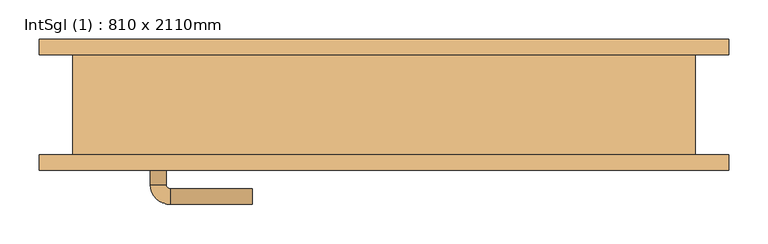
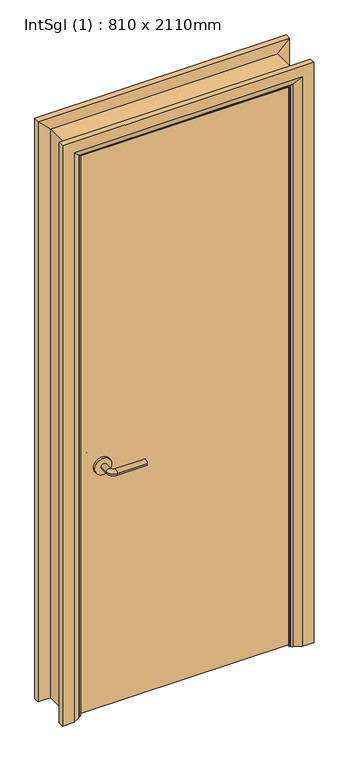
"""IFC4 building model written with IfcOpenShell, lengths in millimetres: door geometry, IntSgl (1) : 810 x 2110mm."""

import ifcopenshell
import ifcopenshell.guid

model = None  # the IFC model being written
_history = None  # IfcOwnerHistory: only IFC2X3 demands one
_inside = {}  # id of a spatial element -> (the spatial element, [elements in it])
_under = {}  # id of a project, library or spatial element -> (it, [spatial elements below it])
_declared = {}  # id of a project -> (the project, [libraries it declares])
_typed = {}  # id of a type object -> (the type object, [elements of that type])
_made_of = {}  # id of a material, layer set ... -> (it, [elements and type objects made of it])


def new_model(schema):
    """Start an empty IFC model of exactly this schema.

    Asked for "IFC4X3", IfcOpenShell would pick the latest addendum, in which some entities
    have other attributes; the version numbers below select the first issue.
    IFC2X3 requires an IfcOwnerHistory on every rooted entity: one is made here for all.
    """
    global model, _history
    if schema == "IFC4X3":
        model = ifcopenshell.file(schema_version=(4, 3, 0, 0))
    else:
        model = ifcopenshell.file(schema=schema)
    _inside.clear()
    _under.clear()
    _declared.clear()
    _typed.clear()
    _made_of.clear()
    _history = None
    if model.schema == "IFC2X3":
        org = make("IfcOrganization", Name="unknown")
        user = make(
            "IfcPersonAndOrganization",
            ThePerson=make("IfcPerson", FamilyName="unknown"),
            TheOrganization=org,
        )
        app = make(
            "IfcApplication",
            ApplicationDeveloper=org,
            Version="unknown",
            ApplicationFullName="unknown",
            ApplicationIdentifier="unknown",
        )
        _history = make(
            "IfcOwnerHistory",
            OwningUser=user,
            OwningApplication=app,
            ChangeAction="ADDED",
            CreationDate=0,
        )
    return model


def make(cls, **values):
    """One entity of the class cls with the attributes given. An attribute that is None is left unset."""
    return model.create_entity(
        cls, **{name: value for name, value in values.items() if value is not None}
    )


def rooted(cls, **values):
    """An entity with a GlobalId (a new one), such as an element, a storey or a relation."""
    return make(cls, GlobalId=ifcopenshell.guid.new(), OwnerHistory=_history, **values)


def si_unit(unit_type, name, prefix=None):
    """IfcSIUnit, for example si_unit("LENGTHUNIT", "METRE", prefix="MILLI")."""
    return make("IfcSIUnit", UnitType=unit_type, Prefix=prefix, Name=name)


def assignment(units):
    """IfcUnitAssignment: the units of a project."""
    return None if units is None else make("IfcUnitAssignment", Units=units)


def point(xyz):
    """IfcCartesianPoint."""
    return None if xyz is None else make("IfcCartesianPoint", Coordinates=xyz)


def direction(xyz):
    """IfcDirection."""
    return None if xyz is None else make("IfcDirection", DirectionRatios=xyz)


def frame(location, z_axis=None, x_axis=None):
    """IfcAxis2Placement3D, a coordinate frame: its origin and axes. An axis left out is left unset."""
    return make(
        "IfcAxis2Placement3D",
        Location=point(location),
        Axis=direction(z_axis),
        RefDirection=direction(x_axis),
    )


def frame_2d(location, x_axis=None):
    """IfcAxis2Placement2D, a coordinate frame in the plane: its origin and x axis."""
    return make(
        "IfcAxis2Placement2D", Location=point(location), RefDirection=direction(x_axis)
    )


def origin():
    """The frame at (0, 0, 0) with its axes left unset."""
    return frame((0.0, 0.0, 0.0))


def place(relative_to, where):
    """IfcLocalPlacement: puts the frame where relative to a parent placement (None: the world)."""
    return make(
        "IfcLocalPlacement", PlacementRelTo=relative_to, RelativePlacement=where
    )


def context(
    kind, dimensions, precision=None, world=None, true_north=None, identifier=None
):
    """IfcGeometricRepresentationContext, for example the 3D "Model" context."""
    return make(
        "IfcGeometricRepresentationContext",
        ContextIdentifier=identifier,
        ContextType=kind,
        CoordinateSpaceDimension=dimensions,
        Precision=precision,
        WorldCoordinateSystem=world,
        TrueNorth=true_north,
    )


def project(units=None, contexts=None):
    """IfcProject with its units and contexts."""
    return rooted(
        "IfcProject",
        Name="project",
        RepresentationContexts=contexts,
        UnitsInContext=assignment(units),
    )


def spatial(cls, under=None, at=None, **own):
    """A site, building, storey or space (cls), placed at a placement, below another one or the project."""
    s = rooted(cls, ObjectPlacement=at, **own)
    if under is not None:
        _under.setdefault(under.id(), (under, []))[1].append(s)
    return s


def polyline(points):
    """IfcPolyline through the points."""
    return make("IfcPolyline", Points=[point(p) for p in points])


def circle_curve(where, radius):
    """IfcCircle in the frame where."""
    return make("IfcCircle", Position=where, Radius=radius)


def ellipse_curve(where, semi_axis1, semi_axis2):
    """IfcEllipse in the frame where."""
    return make(
        "IfcEllipse", Position=where, SemiAxis1=semi_axis1, SemiAxis2=semi_axis2
    )


def trimmed(basis, trim1, trim2, sense, master):
    """IfcTrimmedCurve: the piece of a basis curve between two trims."""
    return make(
        "IfcTrimmedCurve",
        BasisCurve=basis,
        Trim1=trim1,
        Trim2=trim2,
        SenseAgreement=sense,
        MasterRepresentation=master,
    )


def segment(curve, same_sense, transition):
    """IfcCompositeCurveSegment."""
    return make(
        "IfcCompositeCurveSegment",
        Transition=transition,
        SameSense=same_sense,
        ParentCurve=curve,
    )


def composite_curve(segments, self_intersect=None):
    """IfcCompositeCurve: segments joined end to end."""
    return make("IfcCompositeCurve", Segments=segments, SelfIntersect=self_intersect)


def outline(outer, holes=None, kind="AREA"):
    """IfcArbitraryClosedProfileDef: a profile drawn as a closed curve; with holes, ...WithVoids."""
    if holes is None:
        return make("IfcArbitraryClosedProfileDef", ProfileType=kind, OuterCurve=outer)
    return make(
        "IfcArbitraryProfileDefWithVoids",
        ProfileType=kind,
        OuterCurve=outer,
        InnerCurves=holes,
    )


def extrude(swept, where, along, depth):
    """IfcExtrudedAreaSolid: the profile swept, set in the frame where, extruded along a direction by depth."""
    return make(
        "IfcExtrudedAreaSolid",
        SweptArea=swept,
        Position=where,
        ExtrudedDirection=direction(along),
        Depth=depth,
    )


def faces_of(points, faces, orient=None, outer=None):
    """IfcFace entities. A face is a list of loops; a loop is a list of indices into points, from 0.

    orient and outer hold one flag for each loop. By default every Orientation is true, the
    first loop of a face is its IfcFaceOuterBound and the others are IfcFaceBound.
    """
    made = []
    for i, loops in enumerate(faces):
        bounds = []
        for j, loop in enumerate(loops):
            is_outer = j == 0 if outer is None else outer[i][j]
            bounds.append(
                make(
                    "IfcFaceOuterBound" if is_outer else "IfcFaceBound",
                    Bound=make("IfcPolyLoop", Polygon=[points[k] for k in loop]),
                    Orientation=True if orient is None else orient[i][j],
                )
            )
        made.append(make("IfcFace", Bounds=bounds))
    return made


def faceted_brep(points, faces, orient=None, outer=None, voids=None):
    """IfcFacetedBrep: a solid bounded by flat faces; with voids (closed shells), ...WithVoids."""
    shared = [point(p) for p in points]
    hull = make("IfcClosedShell", CfsFaces=faces_of(shared, faces, orient, outer))
    if voids is None:
        return make("IfcFacetedBrep", Outer=hull)
    return make(
        "IfcFacetedBrepWithVoids",
        Outer=hull,
        Voids=[
            make(cls, CfsFaces=faces_of(shared, fs, o, b)) for cls, fs, o, b in voids
        ],
    )


def shape(context_of_items, identifier, shape_type, items):
    """IfcShapeRepresentation: the items that make up one representation, for example the "Body"."""
    return make(
        "IfcShapeRepresentation",
        ContextOfItems=context_of_items,
        RepresentationIdentifier=identifier,
        RepresentationType=shape_type,
        Items=items,
    )


def source(mapping_origin, context_of_items, identifier, shape_type, items):
    """IfcRepresentationMap: a shape defined once, which mapped items show again and again."""
    return make(
        "IfcRepresentationMap",
        MappingOrigin=mapping_origin,
        MappedRepresentation=shape(context_of_items, identifier, shape_type, items),
    )


def transform(
    local_origin,
    x_axis=None,
    y_axis=None,
    z_axis=None,
    scale=None,
    scale2=None,
    scale3=None,
    uniform=True,
):
    """IfcCartesianTransformationOperator3D, or its non-uniform kind. x_axis, y_axis, z_axis: its Axis1, 2, 3."""
    if uniform:
        return make(
            "IfcCartesianTransformationOperator3D",
            Axis1=direction(x_axis),
            Axis2=direction(y_axis),
            LocalOrigin=point(local_origin),
            Scale=scale,
            Axis3=direction(z_axis),
        )
    return make(
        "IfcCartesianTransformationOperator3DnonUniform",
        Axis1=direction(x_axis),
        Axis2=direction(y_axis),
        LocalOrigin=point(local_origin),
        Scale=scale,
        Axis3=direction(z_axis),
        Scale2=scale2,
        Scale3=scale3,
    )


def mapped(mapping_source, mapping_target):
    """IfcMappedItem: shows the shape of a source again, moved by a transform."""
    return make(
        "IfcMappedItem", MappingSource=mapping_source, MappingTarget=mapping_target
    )


def made_of(thing, what):
    """Note that an element or type object is made of a material, layer set ...; save() writes the relation."""
    if what is not None:
        _made_of.setdefault(what.id(), (what, []))[1].append(thing)
    return thing


def element(
    cls,
    number,
    at=None,
    inside=None,
    cuts=None,
    type_object=None,
    material=None,
    context=None,
    identifier="Body",
    shape_type=None,
    held_by="IfcProductDefinitionShape",
    body=None,
    shapes=None,
    **own,
):
    """One element of the class cls, such as IfcWall. Its Tag is "e" and its number.

    at: its placement. inside: the storey or other place that contains it. cuts: it is an
    opening in that element (IfcRelVoidsElement). A single representation is given by context,
    identifier, shape_type and body (its items); several are given by shapes. held_by: the class
    of the entity that holds the representations. save() writes the other relations.
    """
    e = rooted(cls, Tag="e%d" % number, ObjectPlacement=at, **own)
    if body is not None:
        shapes = [shape(context, identifier, shape_type, body)]
    if shapes is not None:
        e.Representation = make(held_by, Representations=shapes)
    if inside is not None:
        _inside.setdefault(inside.id(), (inside, []))[1].append(e)
    if cuts is not None:
        rooted(
            "IfcRelVoidsElement", RelatingBuildingElement=cuts, RelatedOpeningElement=e
        )
    if type_object is not None:
        _typed.setdefault(type_object.id(), (type_object, []))[1].append(e)
    return made_of(e, material)


def aggregate(whole, parts):
    """IfcRelAggregates: a whole, such as a stair, and the parts it consists of."""
    return rooted("IfcRelAggregates", RelatingObject=whole, RelatedObjects=parts)


def save(model, path):
    """Write the relations noted so far, then the file.

    IfcRelAggregates (storeys below a building ...), IfcRelContainedInSpatialStructure (elements
    in a storey), IfcRelDefinesByType, IfcRelAssociatesMaterial and IfcRelDeclares: one each for
    every whole, place, type object, material and project.
    """
    for whole, parts in _under.values():
        aggregate(whole, parts)
    for where, things in _inside.values():
        rooted(
            "IfcRelContainedInSpatialStructure",
            RelatedElements=things,
            RelatingStructure=where,
        )
    for kind, things in _typed.values():
        rooted("IfcRelDefinesByType", RelatedObjects=things, RelatingType=kind)
    for what, things in _made_of.values():
        rooted("IfcRelAssociatesMaterial", RelatedObjects=things, RelatingMaterial=what)
    for by, libraries in _declared.values():
        rooted("IfcRelDeclares", RelatingContext=by, RelatedDefinitions=libraries)
    model.write(path)


def plane_surface(at):
    """IfcPlane: the flat surface through the origin of the frame at, square to its z axis."""
    return make("IfcPlane", Position=at)


def cylinder_surface(at, radius):
    """IfcCylindricalSurface: all points at the distance radius from the z axis of the frame at."""
    return make("IfcCylindricalSurface", Position=at, Radius=radius)


def revolved_surface(curve, axis_point, axis_direction):
    """IfcSurfaceOfRevolution: the curve turned about the line through axis_point along axis_direction."""
    return make(
        "IfcSurfaceOfRevolution",
        SweptCurve=make("IfcArbitraryOpenProfileDef", ProfileType="CURVE", Curve=curve),
        AxisPosition=make("IfcAxis1Placement", Location=point(axis_point), Axis=direction(axis_direction)),
    )


def advanced_brep(points, edges, surfaces, faces):
    """IfcAdvancedBrep: a solid bounded by faces that lie on surfaces and meet in shared edges.

    An edge is (start, end): straight between two places in points (the first is 0);
    or (start, end, curve); or (start, end, curve, False) where it runs against its curve.
    A face is (place in surfaces, loops), or (place, loops, False) where it looks against
    its surface's normal. A loop lists edges by number (the first is 1), with a minus sign
    where the edge is run from its end to its start. The first loop is the outer one.
    """
    corners = [point(p) for p in points]
    vertices = [make("IfcVertexPoint", VertexGeometry=c) for c in corners]
    made = []
    for start, end, *more in edges:
        made.append(
            make(
                "IfcEdgeCurve",
                EdgeStart=vertices[start],
                EdgeEnd=vertices[end],
                EdgeGeometry=more[0] if more else make("IfcPolyline", Points=[corners[start], corners[end]]),
                SameSense=more[1] if len(more) > 1 else True,
            )
        )
    hull = []
    for where, loops, *sense in faces:
        bounds = []
        for j, loop in enumerate(loops):
            ring = [make("IfcOrientedEdge", EdgeElement=made[abs(k) - 1], Orientation=k > 0) for k in loop]
            bounds.append(
                make(
                    "IfcFaceOuterBound" if j == 0 else "IfcFaceBound",
                    Bound=make("IfcEdgeLoop", EdgeList=ring),
                    Orientation=True,
                )
            )
        hull.append(make("IfcAdvancedFace", Bounds=bounds, FaceSurface=surfaces[where], SameSense=sense[0] if sense else True))
    return make("IfcAdvancedBrep", Outer=make("IfcClosedShell", CfsFaces=hull))


def intsgl_1_810_x_2110mm_198b6b43(model_context):
    return source(origin(), model_context, "Body", "SolidModel", [
        advanced_brep(
        [(-298.0, -17.75, 900.0), (-278.0, -17.75, 900.0), (-298.0, 12.25, 900.0), (-278.0, 12.25, 900.0), (-273.0, 17.25, 900.0), (-273.0, 37.25, 900.0), (-168.0, 37.25, 900.0), (-168.0, 17.25, 900.0)],
        [
            (0, 1, circle_curve(frame((-288.0, -17.75, 900.0), z_axis=(0.0, -1.0, 0.0), x_axis=(1.0, 0.0, 0.0)), 10.0)),
            (1, 0, circle_curve(frame((-288.0, -17.75, 900.0), z_axis=(0.0, -1.0, 0.0), x_axis=(1.0, 0.0, 0.0)), 10.0)),
            (0, 2),
            (2, 3, circle_curve(frame((-288.0, 12.25, 900.0), z_axis=(0.0, -1.0, 0.0), x_axis=(1.0, 0.0, 0.0)), 10.0)),
            (3, 1),
            (3, 2, circle_curve(frame((-288.0, 12.25, 900.0), z_axis=(0.0, -1.0, 0.0), x_axis=(1.0, 0.0, 0.0)), 10.0)),
            (4, 3, circle_curve(frame((-273.0, 12.25, 900.0), z_axis=(0.0, 0.0, 1.0), x_axis=(-1.0, 0.0, 0.0)), 5.0)),
            (2, 5, circle_curve(frame((-273.0, 12.25, 900.0), z_axis=(0.0, 0.0, -1.0), x_axis=(-1.0, 0.0, 0.0)), 25.0)),
            (5, 4, circle_curve(frame((-273.0, 27.25, 900.0), z_axis=(-1.0, 0.0, 0.0), x_axis=(0.0, -1.0, 0.0)), 10.0)),
            (4, 5, circle_curve(frame((-273.0, 27.25, 900.0), z_axis=(-1.0, 0.0, 0.0), x_axis=(0.0, -1.0, 0.0)), 10.0)),
            (6, 7, circle_curve(frame((-168.0, 27.25, 900.0), z_axis=(1.0, 0.0, 0.0), x_axis=(0.0, -1.0, 0.0)), 10.0)),
            (7, 6, circle_curve(frame((-168.0, 27.25, 900.0), z_axis=(1.0, 0.0, 0.0), x_axis=(0.0, -1.0, 0.0)), 10.0)),
            (5, 6),
            (7, 4),
        ],
        [
            plane_surface(frame((-288.0, -17.75, 900.0), z_axis=(0.0, -1.0, 0.0), x_axis=(0.0, 0.0, 1.0))),
            cylinder_surface(frame((-288.0, -17.75, 900.0), z_axis=(0.0, -1.0, 0.0), x_axis=(1.0, 0.0, 0.0)), 10.0),
            revolved_surface(trimmed(ellipse_curve(frame((-288.0, 12.25, 900.0), z_axis=(0.0, -1.0, 0.0), x_axis=(1.0, 0.0, 0.0)), 10.0, 10.0), [point((-298.0, 12.25, 900.0))], [point((-278.0, 12.25, 900.0))], True, "CARTESIAN"), (-273.0, 12.25, 900.0), (0.0, 0.0, -1.0)),
            revolved_surface(trimmed(ellipse_curve(frame((-288.0, 12.25, 900.0), z_axis=(0.0, -1.0, 0.0), x_axis=(1.0, 0.0, 0.0)), 10.0, 10.0), [point((-278.0, 12.25, 900.0))], [point((-298.0, 12.25, 900.0))], True, "CARTESIAN"), (-273.0, 12.25, 900.0), (0.0, 0.0, -1.0)),
            plane_surface(frame((-168.0, 27.25, 900.0), z_axis=(1.0, 0.0, 0.0), x_axis=(0.0, 0.0, 1.0))),
            cylinder_surface(frame((-273.0, 27.25, 900.0), z_axis=(-1.0, 0.0, 0.0), x_axis=(0.0, -1.0, 0.0)), 10.0),
        ],
        [
            (0, [[1, 2]]),
            (1, [[-1, 3, 4, 5]]),
            (1, [[-2, -5, 6, -3]]),
            (2, [[7, -4, 8, 9]]),
            (3, [[-8, -6, -7, 10]]),
            (4, [[11, 12]]),
            (5, [[-9, 13, -12, 14]]),
            (5, [[-10, -14, -11, -13]]),
        ],
    ),
        extrude(outline(composite_curve([segment(trimmed(circle_curve(frame_2d((900.0, -290.5)), 30.0), [point((900.0, -320.5))], [point((900.0, -260.5))], False, "CARTESIAN"), True, "CONTINUOUS"), segment(trimmed(circle_curve(frame_2d((900.0, -290.5)), 30.0), [point((900.0, -260.5))], [point((900.0, -320.5))], False, "CARTESIAN"), True, "CONTINUOUS")], self_intersect=False)), frame((0.0, -25.75, 0.0), z_axis=(0.0, 1.0, 0.0), x_axis=(0.0, 0.0, 1.0)), (0.0, 0.0, 1.0), 8.0),
        advanced_brep(
        [(-298.0, -71.75, 900.0), (-278.0, -71.75, 900.0), (-278.0, -101.75, 900.0), (-298.0, -101.75, 900.0), (-273.0, -106.75, 900.0), (-273.0, -126.75, 900.0), (-168.0, -126.75, 900.0), (-168.0, -106.75, 900.0)],
        [
            (0, 1, circle_curve(frame((-288.0, -71.75, 900.0), z_axis=(0.0, 1.0, 0.0), x_axis=(1.0, 0.0, 0.0)), 10.0)),
            (1, 0, circle_curve(frame((-288.0, -71.75, 900.0), z_axis=(0.0, 1.0, 0.0), x_axis=(1.0, 0.0, 0.0)), 10.0)),
            (1, 2),
            (2, 3, circle_curve(frame((-288.0, -101.75, 900.0), z_axis=(0.0, 1.0, 0.0), x_axis=(1.0, 0.0, 0.0)), 10.0)),
            (3, 0),
            (3, 2, circle_curve(frame((-288.0, -101.75, 900.0), z_axis=(0.0, 1.0, 0.0), x_axis=(1.0, 0.0, 0.0)), 10.0)),
            (4, 5, circle_curve(frame((-273.0, -116.75, 900.0), z_axis=(-1.0, 0.0, 0.0), x_axis=(0.0, 1.0, 0.0)), 10.0)),
            (5, 3, circle_curve(frame((-273.0, -101.75, 900.0), z_axis=(0.0, 0.0, -1.0), x_axis=(-1.0, 0.0, 0.0)), 25.0)),
            (2, 4, circle_curve(frame((-273.0, -101.75, 900.0), z_axis=(0.0, 0.0, 1.0), x_axis=(-1.0, 0.0, 0.0)), 5.0)),
            (5, 4, circle_curve(frame((-273.0, -116.75, 900.0), z_axis=(-1.0, 0.0, 0.0), x_axis=(0.0, 1.0, 0.0)), 10.0)),
            (6, 7, circle_curve(frame((-168.0, -116.75, 900.0), z_axis=(1.0, 0.0, 0.0), x_axis=(0.0, 1.0, 0.0)), 10.0)),
            (7, 6, circle_curve(frame((-168.0, -116.75, 900.0), z_axis=(1.0, 0.0, 0.0), x_axis=(0.0, 1.0, 0.0)), 10.0)),
            (4, 7),
            (6, 5),
        ],
        [
            plane_surface(frame((-288.0, -71.75, 900.0), z_axis=(0.0, 1.0, 0.0), x_axis=(0.0, 0.0, 1.0))),
            cylinder_surface(frame((-288.0, -71.75, 900.0), z_axis=(0.0, 1.0, 0.0), x_axis=(1.0, 0.0, 0.0)), 10.0),
            revolved_surface(trimmed(ellipse_curve(frame((-288.0, -101.75, 900.0), z_axis=(0.0, -1.0, 0.0), x_axis=(1.0, 0.0, 0.0)), 10.0, 10.0), [point((-298.0, -101.75, 900.0))], [point((-278.0, -101.75, 900.0))], True, "CARTESIAN"), (-273.0, -101.75, 900.0), (0.0, 0.0, -1.0)),
            revolved_surface(trimmed(ellipse_curve(frame((-288.0, -101.75, 900.0), z_axis=(0.0, -1.0, 0.0), x_axis=(1.0, 0.0, 0.0)), 10.0, 10.0), [point((-278.0, -101.75, 900.0))], [point((-298.0, -101.75, 900.0))], True, "CARTESIAN"), (-273.0, -101.75, 900.0), (0.0, 0.0, -1.0)),
            plane_surface(frame((-168.0, -116.75, 900.0), z_axis=(1.0, 0.0, 0.0), x_axis=(0.0, 0.0, 1.0))),
            cylinder_surface(frame((-273.0, -116.75, 900.0), z_axis=(-1.0, 0.0, 0.0), x_axis=(0.0, 1.0, 0.0)), 10.0),
        ],
        [
            (0, [[1, 2]]),
            (1, [[3, 4, 5, -2]]),
            (1, [[-5, 6, -3, -1]]),
            (2, [[7, 8, -4, 9]]),
            (3, [[10, -9, -6, -8]]),
            (4, [[11, 12]]),
            (5, [[13, -11, 14, -7]]),
            (5, [[-14, -12, -13, -10]]),
        ],
    ),
        extrude(outline(composite_curve([segment(trimmed(circle_curve(frame_2d((900.0, -290.5)), 30.0), [point((900.0, -320.5))], [point((900.0, -260.5))], False, "CARTESIAN"), True, "CONTINUOUS"), segment(trimmed(circle_curve(frame_2d((900.0, -290.5)), 30.0), [point((900.0, -260.5))], [point((900.0, -320.5))], False, "CARTESIAN"), True, "CONTINUOUS")], self_intersect=False)), frame((0.0, -71.75, 0.0), z_axis=(0.0, 1.0, 0.0), x_axis=(0.0, 0.0, 1.0)), (0.0, 0.0, 1.0), 8.0),
        extrude(outline(polyline([(363.0, -25.75), (363.0, -63.75), (-363.0, -63.75), (-363.0, -25.75), (363.0, -25.75)])), frame((0.0, 0.0, 8.0), z_axis=(0.0, 0.0, 1.0), x_axis=(1.0, 0.0, 0.0)), (0.0, 0.0, 1.0), 2060.0),
        advanced_brep(
        [(440.0, -83.75, 0.0), (400.0, -83.75, 0.0), (374.0, -69.75, 0.0), (370.0, -63.75, 0.0), (440.0, -63.75, 0.0), (440.0, -63.75, 2145.0), (440.0, -83.75, 2145.0), (370.0, -63.75, 2075.0), (-370.0, -63.75, 2075.0), (-370.0, -63.75, 0.0), (-440.0, -63.75, 0.0), (-440.0, -63.75, 2145.0), (374.0, -69.75, 2079.0), (400.0, -83.75, 2105.0), (-440.0, -83.75, 2145.0), (-440.0, -83.75, 0.0), (-400.0, -83.75, 0.0), (-400.0, -83.75, 2105.0), (-374.0, -69.75, 2079.0), (-374.0, -69.75, 0.0)],
        [
            (0, 1),
            (1, 2),
            (2, 3, circle_curve(frame((378.0, -62.75, 0.0), z_axis=(0.0, 0.0, -1.0), x_axis=(1.0, 0.0, 0.0)), 8.0622577)),
            (3, 4),
            (4, 0),
            (4, 5),
            (5, 6),
            (6, 0),
            (3, 7),
            (7, 8),
            (8, 9),
            (9, 10),
            (10, 11),
            (11, 5),
            (2, 12),
            (12, 7, ellipse_curve(frame((378.0, -62.75, 2083.0), z_axis=(0.7071067811865475, 0.0, -0.7071067811865475), x_axis=(-0.7071067811865474, 0.0, -0.7071067811865476)), 11.4017543, 8.0622577)),
            (1, 13),
            (13, 12),
            (6, 14),
            (14, 15),
            (15, 16),
            (16, 17),
            (17, 13),
            (11, 14),
            (12, 18),
            (18, 8, ellipse_curve(frame((-378.0, -62.75, 2083.0), z_axis=(0.7071067811865475, 0.0, 0.7071067811865475), x_axis=(0.7071067811865476, 0.0, -0.7071067811865474)), 11.4017543, 8.0622577)),
            (17, 18),
            (15, 10),
            (9, 19, circle_curve(frame((-378.0, -62.75, 0.0), z_axis=(0.0, 0.0, -1.0), x_axis=(-1.0, 0.0, 0.0)), 8.0622577)),
            (19, 16),
            (18, 19),
        ],
        [
            plane_surface(frame((370.0, -63.75, 0.0), z_axis=(0.0, 0.0, -1.0), x_axis=(0.0, 1.0, 0.0))),
            plane_surface(frame((440.0, -83.75, 0.0), z_axis=(1.0, 0.0, 0.0), x_axis=(0.0, 0.0, 1.0))),
            plane_surface(frame((440.0, -63.75, 0.0), z_axis=(0.0, 1.0, 0.0), x_axis=(0.0, 0.0, 1.0))),
            cylinder_surface(frame((378.0, -62.75, 0.0), z_axis=(0.0, 0.0, -1.0), x_axis=(1.0, 0.0, 0.0)), 8.0622577),
            plane_surface(frame((374.0, -69.75, 0.0), z_axis=(-0.4740998230350126, -0.880471099922178, 0.0), x_axis=(0.0, 0.0, 1.0))),
            plane_surface(frame((400.0, -83.75, 0.0), z_axis=(0.0, -1.0, 0.0), x_axis=(0.0, 0.0, 1.0))),
            plane_surface(frame((440.0, -83.75, 2145.0), z_axis=(0.0, 0.0, 1.0), x_axis=(-1.0, 0.0, 0.0))),
            cylinder_surface(frame((370.0, -62.75, 2083.0), z_axis=(1.0, 0.0, 0.0), x_axis=(0.0, 0.0, 1.0)), 8.0622577),
            plane_surface(frame((374.0, -69.75, 2079.0), z_axis=(0.0, -0.8804710999221764, -0.4740998230350154), x_axis=(-1.0, 0.0, 0.0))),
            plane_surface(frame((-370.0, -63.75, 0.0), z_axis=(0.0, 0.0, -1.0), x_axis=(0.0, 1.0, 0.0))),
            plane_surface(frame((-440.0, -83.75, 2145.0), z_axis=(-1.0, 0.0, 0.0), x_axis=(0.0, 0.0, -1.0))),
            cylinder_surface(frame((-378.0, -62.75, 2075.0), z_axis=(0.0, 0.0, 1.0), x_axis=(-1.0, 0.0, 0.0)), 8.0622577),
            plane_surface(frame((-374.0, -69.75, 2079.0), z_axis=(0.47409982303501824, -0.8804710999221749, 0.0), x_axis=(0.0, 0.0, -1.0))),
        ],
        [
            (0, [[1, 2, 3, 4, 5]]),
            (1, [[6, 7, 8, -5]]),
            (2, [[9, 10, 11, 12, 13, 14, -6, -4]]),
            (3, [[15, 16, -9, -3]]),
            (4, [[17, 18, -15, -2]]),
            (5, [[-8, 19, 20, 21, 22, 23, -17, -1]]),
            (6, [[-14, 24, -19, -7]]),
            (7, [[25, 26, -10, -16]]),
            (8, [[-23, 27, -25, -18]]),
            (9, [[28, -12, 29, 30, -21]]),
            (10, [[-13, -28, -20, -24]]),
            (11, [[31, -29, -11, -26]]),
            (12, [[-22, -30, -31, -27]]),
        ],
    ),
        extrude(outline(polyline([(0.0, -346.0), (2051.0, -346.0), (2051.0, 346.0), (0.0, 346.0), (0.0, 365.0), (2070.0, 365.0), (2070.0, -365.0), (0.0, -365.0), (0.0, -346.0)])), frame((0.0, -23.75, 0.0), z_axis=(0.0, 1.0, 0.0), x_axis=(0.0, 0.0, 1.0)), (0.0, 0.0, 1.0), 32.0),
        advanced_brep(
        [(-440.0, 83.75, 0.0), (-400.0, 83.75, 0.0), (-374.0, 69.75, 0.0), (-370.0, 63.75, 0.0), (-440.0, 63.75, 0.0), (-440.0, 63.75, 2145.0), (-440.0, 83.75, 2145.0), (-370.0, 63.75, 2075.0), (-374.0, 69.75, 2079.0), (-400.0, 83.75, 2105.0), (440.0, 63.75, 2145.0), (440.0, 83.75, 2145.0), (370.0, 63.75, 2075.0), (374.0, 69.75, 2079.0), (400.0, 83.75, 2105.0), (440.0, 83.75, 0.0), (440.0, 63.75, 0.0), (370.0, 63.75, 0.0), (374.0, 69.75, 0.0), (400.0, 83.75, 0.0)],
        [
            (0, 1),
            (1, 2),
            (2, 3, circle_curve(frame((-378.0, 62.75, 0.0), z_axis=(0.0, 0.0, -1.0), x_axis=(-1.0, 0.0, 0.0)), 8.0622577)),
            (3, 4),
            (4, 0),
            (4, 5),
            (5, 6),
            (6, 0),
            (3, 7),
            (7, 5),
            (2, 8),
            (8, 7, ellipse_curve(frame((-378.0, 62.75, 2083.0), z_axis=(-0.7071067811865475, 0.0, -0.7071067811865475), x_axis=(0.7071067811865474, 0.0, -0.7071067811865476)), 11.4017543, 8.0622577)),
            (1, 9),
            (9, 8),
            (6, 9),
            (5, 10),
            (10, 11),
            (11, 6),
            (7, 12),
            (12, 10),
            (8, 13),
            (13, 12, ellipse_curve(frame((378.0, 62.75, 2083.0), z_axis=(-0.7071067811865475, 0.0, 0.7071067811865475), x_axis=(-0.7071067811865476, 0.0, -0.7071067811865474)), 11.4017543, 8.0622577)),
            (9, 14),
            (14, 13),
            (11, 14),
            (15, 16),
            (16, 17),
            (17, 18, circle_curve(frame((378.0, 62.75, 0.0), z_axis=(0.0, 0.0, -1.0), x_axis=(1.0, 0.0, 0.0)), 8.0622577)),
            (18, 19),
            (19, 15),
            (10, 16),
            (15, 11),
            (12, 17),
            (13, 18),
            (14, 19),
        ],
        [
            plane_surface(frame((-370.0, 136.5510989, 0.0), z_axis=(0.0, 0.0, -1.0), x_axis=(1.0, 0.0, 0.0))),
            plane_surface(frame((-440.0, 83.75, 0.0), z_axis=(-1.0, 0.0, 0.0), x_axis=(0.0, 0.0, 1.0))),
            plane_surface(frame((-440.0, 63.75, 0.0), z_axis=(0.0, -1.0, 0.0), x_axis=(0.0, 0.0, 1.0))),
            cylinder_surface(frame((-378.0, 62.75, 0.0), z_axis=(0.0, 0.0, -1.0), x_axis=(-1.0, 0.0, 0.0)), 8.0622577),
            plane_surface(frame((-374.0, 69.75, 0.0), z_axis=(0.4740998230350183, 0.8804710999221749, 0.0), x_axis=(0.0, 0.0, 1.0))),
            plane_surface(frame((-400.0, 83.75, 0.0), z_axis=(0.0, 1.0, 0.0), x_axis=(0.0, 0.0, 1.0))),
            plane_surface(frame((-440.0, 83.75, 2145.0), z_axis=(0.0, 0.0, 1.0), x_axis=(1.0, 0.0, 0.0))),
            plane_surface(frame((-440.0, 63.75, 2145.0), z_axis=(0.0, -1.0, 0.0), x_axis=(1.0, 0.0, 0.0))),
            cylinder_surface(frame((-370.0, 62.75, 2083.0), z_axis=(-1.0, 0.0, 0.0), x_axis=(0.0, 0.0, 1.0)), 8.0622577),
            plane_surface(frame((-374.0, 69.75, 2079.0), z_axis=(0.0, 0.8804710999221749, -0.4740998230350183), x_axis=(1.0, 0.0, 0.0))),
            plane_surface(frame((-400.0, 83.75, 2105.0), z_axis=(0.0, 1.0, 0.0), x_axis=(1.0, 0.0, 0.0))),
            plane_surface(frame((370.0, 136.5510989, 0.0), z_axis=(0.0, 0.0, -1.0), x_axis=(-1.0, 0.0, 0.0))),
            plane_surface(frame((440.0, 83.75, 2145.0), z_axis=(1.0, 0.0, 0.0), x_axis=(0.0, 0.0, -1.0))),
            plane_surface(frame((440.0, 63.75, 2145.0), z_axis=(0.0, -1.0, 0.0), x_axis=(0.0, 0.0, -1.0))),
            cylinder_surface(frame((378.0, 62.75, 2075.0), z_axis=(0.0, 0.0, 1.0), x_axis=(1.0, 0.0, 0.0)), 8.0622577),
            plane_surface(frame((374.0, 69.75, 2079.0), z_axis=(-0.4740998230350183, 0.8804710999221749, 0.0), x_axis=(0.0, 0.0, -1.0))),
            plane_surface(frame((400.0, 83.75, 2105.0), z_axis=(0.0, 1.0, 0.0), x_axis=(0.0, 0.0, -1.0))),
        ],
        [
            (0, [[1, 2, 3, 4, 5]]),
            (1, [[6, 7, 8, -5]]),
            (2, [[9, 10, -6, -4]]),
            (3, [[11, 12, -9, -3]]),
            (4, [[13, 14, -11, -2]]),
            (5, [[-8, 15, -13, -1]]),
            (6, [[16, 17, 18, -7]]),
            (7, [[19, 20, -16, -10]]),
            (8, [[21, 22, -19, -12]]),
            (9, [[23, 24, -21, -14]]),
            (10, [[-18, 25, -23, -15]]),
            (11, [[26, 27, 28, 29, 30]]),
            (12, [[31, -26, 32, -17]]),
            (13, [[33, -27, -31, -20]]),
            (14, [[34, -28, -33, -22]]),
            (15, [[35, -29, -34, -24]]),
            (16, [[-32, -30, -35, -25]]),
        ],
    ),
        faceted_brep([(-365.0, -63.75, 0.0), (-397.0, -63.75, 0.0), (-397.0, 63.75, 0.0), (-365.0, 63.75, 0.0), (-365.0, 63.75, 2070.0), (-365.0, -63.75, 2070.0), (-397.0, 63.75, 2102.0), (-397.0, -63.75, 2102.0), (365.0, 63.75, 2070.0), (365.0, -63.75, 2070.0), (397.0, 63.75, 2102.0), (397.0, -63.75, 2102.0), (365.0, -63.75, 0.0), (365.0, 63.75, 0.0), (397.0, 63.75, 0.0), (397.0, -63.75, 0.0)], [[[0, 1, 2, 3]], [[3, 4, 5, 0]], [[2, 6, 4, 3]], [[1, 7, 6, 2]], [[0, 5, 7, 1]], [[4, 8, 9, 5]], [[6, 10, 8, 4]], [[7, 11, 10, 6]], [[5, 9, 11, 7]], [[12, 13, 14, 15]], [[8, 13, 12, 9]], [[10, 14, 13, 8]], [[11, 15, 14, 10]], [[9, 12, 15, 11]]]),
    ])


if __name__ == "__main__":
    model = new_model("IFC4")
    model_context = context("Model", 3, world=origin())
    ifc_project = project(units=[si_unit("LENGTHUNIT", "METRE", prefix="MILLI")], contexts=[model_context])
    site = spatial("IfcSite", under=ifc_project)
    building = spatial("IfcBuilding", under=site)
    placement = place(None, origin())
    intsgl_1_810_x_2110mm_shape = intsgl_1_810_x_2110mm_198b6b43(model_context)
    element("IfcDoor", 1, ObjectType="IntSgl (1) : 810 x 2110mm", at=placement, inside=building, context=model_context, shape_type="MappedRepresentation", body=[
        mapped(intsgl_1_810_x_2110mm_shape, transform((0.0, 0.0, 0.0), x_axis=(1.0, 0.0, 0.0), y_axis=(0.0, 1.0, 0.0), z_axis=(0.0, 0.0, 1.0))),
    ])
    save(model, "model.ifc")

# Revit data of these elements
# Type "IntSgl (1) : 810 x 2110mm"
#   Construction Type Id = "MDOOR"
#   Analytic Construction = "Metal"
#   Type Mark = "42"
#   Type Comments = "Internal Single"
#   Operation = "SingleSwingRight"
#   Manufacturer = "Revit"
#   Keynote = "L20"
#   Description = "Internal Single Door"
#   Visual Light Transmittance = 0
#   Solar Heat Gain Coefficient = 0
#   Heat Transfer Coefficient (U) = 3.7021 W/(m²·K)
#   UnderCut = 8 mm
#   Tolerance = 2 mm
#   Thickness = 38 mm
#   Structural Tolerance = 8 mm
#   StopDepth = 32 mm
#   Stop Thickness = 19 mm
#   Rough Width = 810 mm
#   Rough Height = 2110 mm
#   Height to Top Lock Rail = 1000 mm
#   Handle Z Distance = 900 mm
#   Handle X Distance = 75 mm
#   Frame Thickness = 32 mm
#   Door Panel Width = 726 mm
#   Door Panel Thickness = 38 mm
#   Door Panel Offset = 0 mm
#   Height = 2110 mm
#   Width = 810 mm
#   Door Panel Height = 2060 mm
#   Architrave Setback = 5 mm
#   Function = 0
#   Vis - Ironmongery = yes
#   Material Ironmongery = Door - Handle
#   Material Frame = Door - Frame/Mullion (1)
#   Material Door = Door - Panel
#   Material Architrave = Door - Architrave
#   Wall Closure = (empty or 0)
# Element 1 (IfcDoor, "IntSgl (1) : 810 x 2110mm")
#   Materials on its faces: "Door - Architrave", "Door - Handle", "Door - Frame/Mullion (1)", "Door - Panel"
# Materials
#   "Door - Handle": class "Miscellaneous", colour RGB 0 0 0, transparency 0, Keynote = "P21"
#   "Door - Frame/Mullion (1)": class "Wood", colour RGB 212 179 113, transparency 0, Keynote = "L20", Cost = 0
#   "Door - Panel": class "Wood", colour RGB 210 159 95, transparency 0, Keynote = "L20"
#   "Door - Architrave": class "Wood", colour RGB 154 90 5, transparency 0, Keynote = "P20"
